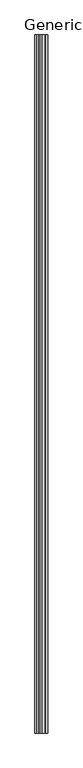
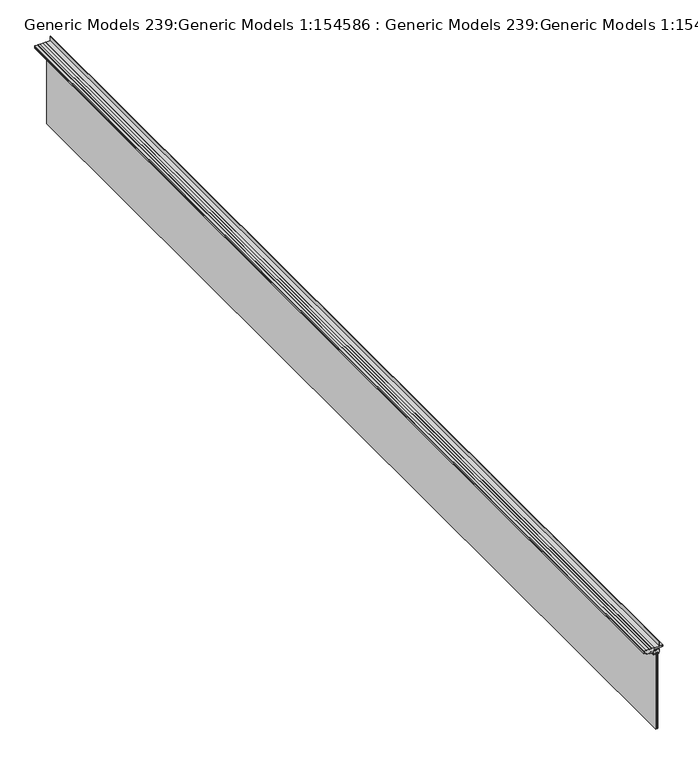
"""IFC4 building model written with IfcOpenShell, lengths in millimetres: proxy geometry, Generic Models 239:Generic Models 1:154586 : Generic Models 239:Generic Models 1:154586."""

from ifc_helpers import new_model, si_unit, point, frame, frame_2d, origin, place, context, project, spatial, polyline, circle_curve, trimmed, segment, composite_curve, outline, extrude, source, transform, mapped, element, save


def generic_models_239_generic_models_1_154586_generic_models_416130f7(model_context):
    return source(origin(), model_context, "Body", "SweptSolid", [
        extrude(outline(polyline([(1586.584463, 8383.5218843), (1586.584463, 496.8218843), (1581.821963, 496.8218843), (1581.821963, 8383.5218843), (1586.584463, 8383.5218843)])), frame((0.0, 0.0, 2290.2205773), z_axis=(0.0, 0.0, 1.0), x_axis=(1.0, 0.0, 0.0)), (0.0, 0.0, 1.0), 602.3375481),
        extrude(outline(polyline([(1581.028213, 8383.5218843), (1581.028213, 496.8218843), (1574.679131, 496.8218843), (1574.679131, 8383.5218843), (1581.028213, 8383.5218843)])), frame((0.0, 0.0, 2886.2081253), z_axis=(0.0, 0.0, 1.0), x_axis=(1.0, 0.0, 0.0)), (0.0, 0.0, 1.0), 6.35),
        extrude(outline(composite_curve([segment(polyline([(2889.7712565, 1587.378213), (2888.7481145, 1588.4013551), (2884.5126753, 1588.4013551), (2884.5126753, 1589.537213), (2882.4863015, 1589.537213), (2882.6758518, 1591.9802525), (2890.4816753, 1594.515613), (2890.4816753, 1596.903213), (2912.7828753, 1596.903213)]), True, "CONTINUOUS"), segment(trimmed(circle_curve(frame_2d((2912.7828753, 1594.515613)), 2.3876), [point((2912.7828753, 1596.903213))], [point((2915.1704753, 1594.515613))], False, "CARTESIAN"), True, "CONTINUOUS"), segment(polyline([(2915.1704753, 1594.515613), (2915.1704753, 1591.950213), (2913.1384753, 1591.950213), (2913.1384753, 1590.273813), (2909.8364753, 1590.273813), (2909.8364753, 1588.368813), (2917.7612753, 1588.368813), (2917.7612753, 1582.755413), (2912.4526753, 1582.755413), (2912.4526753, 1570.563413)]), True, "CONTINUOUS"), segment(trimmed(circle_curve(frame_2d((2912.4526753, 1568.582213)), 1.9812), [point((2912.4526753, 1570.563413))], [point((2912.4526753, 1566.601013))], True, "CARTESIAN"), True, "CONTINUOUS"), segment(polyline([(2912.4526753, 1566.601013), (2912.4526753, 1553.266013)]), True, "CONTINUOUS"), segment(trimmed(circle_curve(frame_2d((2911.6398753, 1553.266013)), 0.8128), [point((2912.4526753, 1553.266013))], [point((2911.6398753, 1552.453213))], False, "CARTESIAN"), True, "CONTINUOUS"), segment(polyline([(2911.6398753, 1552.453213), (2893.3518753, 1552.453213), (2893.3518753, 1554.333731), (2891.7509865, 1554.333731), (2891.7509865, 1552.733531), (2884.2071865, 1552.733531), (2884.2071865, 1556.5014505), (2882.0448365, 1556.5014505), (2881.0321865, 1568.329131), (2890.9635865, 1568.329131), (2893.3518753, 1565.9408422), (2893.3518753, 1587.378213), (2889.7712565, 1587.378213)]), True, "CONTINUOUS")], self_intersect=False)), frame((0.0, 496.8218843, 0.0), z_axis=(0.0, 1.0, 0.0), x_axis=(0.0, 0.0, 1.0)), (0.0, 0.0, 1.0), 7886.7),
        extrude(outline(composite_curve([segment(polyline([(2937.6050253, 1498.7668061), (2937.6050253, 1480.6982627), (2929.6548081, 1480.6982627), (2929.6548081, 1488.6484557), (2927.6736306, 1488.6484557), (2927.6736306, 1480.6982627), (2917.7422116, 1480.6982627), (2917.7422116, 1491.0106177), (2916.929422, 1491.7980696), (2916.929422, 1494.9730696), (2912.9670185, 1494.9730696), (2912.9670185, 1496.5732627), (2909.7920185, 1500.5102316), (2909.7920185, 1502.1104247), (2907.404422, 1502.1104247), (2907.404422, 1521.1604247), (2901.0725895, 1521.1604247), (2901.0725895, 1550.5736487), (2904.2475895, 1550.5736487), (2904.2475895, 1547.5256758), (2912.9343895, 1547.5256758), (2912.9343895, 1529.9996758), (2915.2203895, 1529.9996758), (2915.2203895, 1547.5256758), (2916.160186, 1547.5256758), (2916.160186, 1555.9330115), (2924.1103791, 1555.9330115), (2924.1103791, 1557.9142859), (2917.6914395, 1557.9142859), (2917.6914395, 1561.927413), (2922.5682321, 1561.927413), (2922.5682321, 1596.877813), (2924.990602, 1624.741613), (2933.9220253, 1624.741613), (2933.9220253, 1616.8380474), (2936.2080253, 1616.8380474), (2936.2080253, 1623.1880474), (2937.6050253, 1623.1880474), (2937.6050253, 1598.300213), (2972.9721123, 1598.300213)]), True, "CONTINUOUS"), segment(trimmed(circle_curve(frame_2d((2972.974572, 1597.6017132)), 0.6985041), [point((2972.9721123, 1598.300213))], [point((2972.9769129, 1596.903213))], False, "CARTESIAN"), True, "CONTINUOUS"), segment(polyline([(2972.9769129, 1596.903213), (2937.6050253, 1596.903213), (2937.6050253, 1560.4340452), (2934.4300253, 1560.4340452), (2934.4300253, 1558.1480452), (2937.6050253, 1558.1480452), (2937.6050253, 1541.0486627), (2935.5222253, 1541.0486627), (2935.5222253, 1537.8736627), (2937.6050253, 1537.8736627), (2937.6050253, 1520.846563), (2934.4300253, 1520.846563), (2934.4300253, 1518.5605591), (2937.6050253, 1518.5605591), (2937.6050253, 1501.05281), (2934.4300253, 1501.05281), (2934.4300253, 1498.7668061), (2937.6050253, 1498.7668061)]), True, "CONTINUOUS")], self_intersect=False)), frame((0.0, 496.8218843, 0.0), z_axis=(0.0, 1.0, 0.0), x_axis=(0.0, 0.0, 1.0)), (0.0, 0.0, 1.0), 7886.7),
        extrude(outline(polyline([(1573.885381, 8383.5218843), (1573.885381, 496.8218843), (1569.122881, 496.8218843), (1569.122881, 8383.5218843), (1573.885381, 8383.5218843)])), frame((0.0, 0.0, 2290.2205773), z_axis=(0.0, 0.0, 1.0), x_axis=(1.0, 0.0, 0.0)), (0.0, 0.0, 1.0), 602.3375481),
    ])


if __name__ == "__main__":
    model = new_model("IFC4")
    model_context = context("Model", 3, world=origin())
    ifc_project = project(units=[si_unit("LENGTHUNIT", "METRE", prefix="MILLI")], contexts=[model_context])
    site = spatial("IfcSite", under=ifc_project)
    building = spatial("IfcBuilding", under=site)
    placement = place(None, origin())
    generic_models_239_generic_models_1_154586_generic_models_shape = generic_models_239_generic_models_1_154586_generic_models_416130f7(model_context)
    element("IfcBuildingElementProxy", 1, Name="Generic Models 239:Generic Models 1:154586 : Generic Models 239:Generic Models 1:154586", ObjectType="Generic Models 239:Generic Models 1:154586 : Generic Models 239:Generic Models 1:154586", at=placement, inside=building, context=model_context, shape_type="MappedRepresentation", body=[
        mapped(generic_models_239_generic_models_1_154586_generic_models_shape, transform((0.0, 0.0, 0.0), x_axis=(1.0, 0.0, 0.0), y_axis=(0.0, 1.0, 0.0), z_axis=(0.0, 0.0, 1.0))),
    ])
    save(model, "model.ifc")

# Revit data of these elements
# Type "Generic Models 239:Generic Models 1:154586 : Generic Models 239:Generic Models 1:154586"
#   NameOverride = "Generic Models 239:Generic Models 1:154586"
#   ObjectTypeOverride = "Generic Models 239:Generic Models 1"
#   Reference = "Generic Models 1"
#   Category = "Generic Models"
#   Tag = "154586"
# Element 1 (IfcBuildingElementProxy, "Generic Models 239:Generic Models 1:154586 : Generic Models 239:Generic Models 1:154586")
#   Materials on its faces: "_WINDOW PER SCHEDULE 24593"
# Materials
#   "_WINDOW PER SCHEDULE 24593": class "Unassigned", colour RGB 255 255 255, transparency 0
